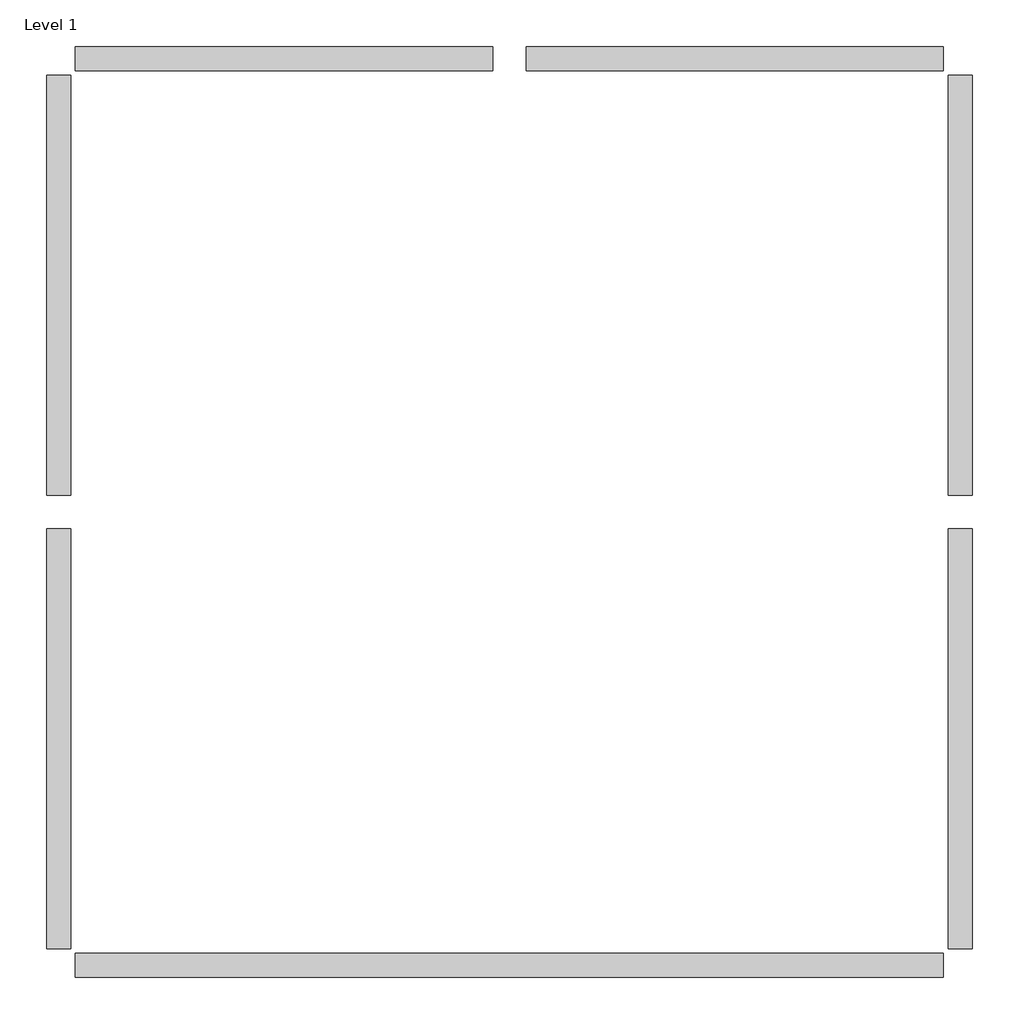
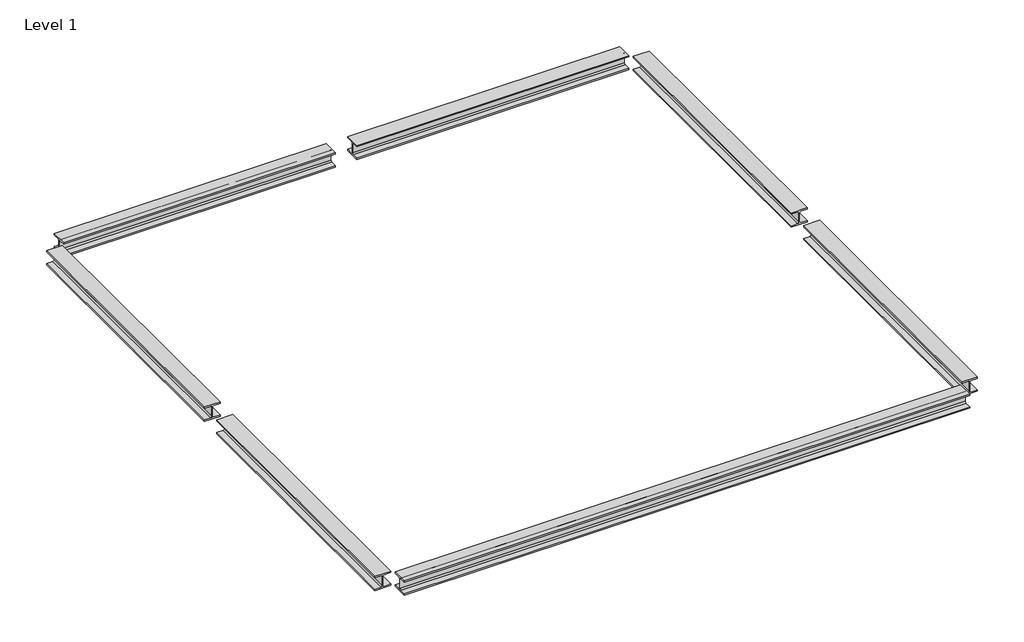
# One storey: 7 beams.
"""IFC4 building model written with IfcOpenShell, lengths in millimetres."""

import ifcopenshell
import ifcopenshell.guid

model = None  # the IFC model being written
_history = None  # IfcOwnerHistory: only IFC2X3 demands one
_inside = {}  # id of a spatial element -> (the spatial element, [elements in it])
_under = {}  # id of a project, library or spatial element -> (it, [spatial elements below it])
_declared = {}  # id of a project -> (the project, [libraries it declares])
_typed = {}  # id of a type object -> (the type object, [elements of that type])
_made_of = {}  # id of a material, layer set ... -> (it, [elements and type objects made of it])


def new_model(schema):
    """Start an empty IFC model of exactly this schema.

    Asked for "IFC4X3", IfcOpenShell would pick the latest addendum, in which some entities
    have other attributes; the version numbers below select the first issue.
    IFC2X3 requires an IfcOwnerHistory on every rooted entity: one is made here for all.
    """
    global model, _history
    if schema == "IFC4X3":
        model = ifcopenshell.file(schema_version=(4, 3, 0, 0))
    else:
        model = ifcopenshell.file(schema=schema)
    _inside.clear()
    _under.clear()
    _declared.clear()
    _typed.clear()
    _made_of.clear()
    _history = None
    if model.schema == "IFC2X3":
        org = make("IfcOrganization", Name="unknown")
        user = make(
            "IfcPersonAndOrganization",
            ThePerson=make("IfcPerson", FamilyName="unknown"),
            TheOrganization=org,
        )
        app = make(
            "IfcApplication",
            ApplicationDeveloper=org,
            Version="unknown",
            ApplicationFullName="unknown",
            ApplicationIdentifier="unknown",
        )
        _history = make(
            "IfcOwnerHistory",
            OwningUser=user,
            OwningApplication=app,
            ChangeAction="ADDED",
            CreationDate=0,
        )
    return model


def make(cls, **values):
    """One entity of the class cls with the attributes given. An attribute that is None is left unset."""
    return model.create_entity(
        cls, **{name: value for name, value in values.items() if value is not None}
    )


def rooted(cls, **values):
    """An entity with a GlobalId (a new one), such as an element, a storey or a relation."""
    return make(cls, GlobalId=ifcopenshell.guid.new(), OwnerHistory=_history, **values)


def si_unit(unit_type, name, prefix=None):
    """IfcSIUnit, for example si_unit("LENGTHUNIT", "METRE", prefix="MILLI")."""
    return make("IfcSIUnit", UnitType=unit_type, Prefix=prefix, Name=name)


def assignment(units):
    """IfcUnitAssignment: the units of a project."""
    return None if units is None else make("IfcUnitAssignment", Units=units)


def point(xyz):
    """IfcCartesianPoint."""
    return None if xyz is None else make("IfcCartesianPoint", Coordinates=xyz)


def direction(xyz):
    """IfcDirection."""
    return None if xyz is None else make("IfcDirection", DirectionRatios=xyz)


def frame(location, z_axis=None, x_axis=None):
    """IfcAxis2Placement3D, a coordinate frame: its origin and axes. An axis left out is left unset."""
    return make(
        "IfcAxis2Placement3D",
        Location=point(location),
        Axis=direction(z_axis),
        RefDirection=direction(x_axis),
    )


def frame_2d(location, x_axis=None):
    """IfcAxis2Placement2D, a coordinate frame in the plane: its origin and x axis."""
    return make(
        "IfcAxis2Placement2D", Location=point(location), RefDirection=direction(x_axis)
    )


def origin():
    """The frame at (0, 0, 0) with its axes left unset."""
    return frame((0.0, 0.0, 0.0))


def place(relative_to, where):
    """IfcLocalPlacement: puts the frame where relative to a parent placement (None: the world)."""
    return make(
        "IfcLocalPlacement", PlacementRelTo=relative_to, RelativePlacement=where
    )


def context(
    kind, dimensions, precision=None, world=None, true_north=None, identifier=None
):
    """IfcGeometricRepresentationContext, for example the 3D "Model" context."""
    return make(
        "IfcGeometricRepresentationContext",
        ContextIdentifier=identifier,
        ContextType=kind,
        CoordinateSpaceDimension=dimensions,
        Precision=precision,
        WorldCoordinateSystem=world,
        TrueNorth=true_north,
    )


def project(units=None, contexts=None):
    """IfcProject with its units and contexts."""
    return rooted(
        "IfcProject",
        Name="project",
        RepresentationContexts=contexts,
        UnitsInContext=assignment(units),
    )


def spatial(cls, under=None, at=None, **own):
    """A site, building, storey or space (cls), placed at a placement, below another one or the project."""
    s = rooted(cls, ObjectPlacement=at, **own)
    if under is not None:
        _under.setdefault(under.id(), (under, []))[1].append(s)
    return s


def polyline(points):
    """IfcPolyline through the points."""
    return make("IfcPolyline", Points=[point(p) for p in points])


def circle_curve(where, radius):
    """IfcCircle in the frame where."""
    return make("IfcCircle", Position=where, Radius=radius)


def trimmed(basis, trim1, trim2, sense, master):
    """IfcTrimmedCurve: the piece of a basis curve between two trims."""
    return make(
        "IfcTrimmedCurve",
        BasisCurve=basis,
        Trim1=trim1,
        Trim2=trim2,
        SenseAgreement=sense,
        MasterRepresentation=master,
    )


def segment(curve, same_sense, transition):
    """IfcCompositeCurveSegment."""
    return make(
        "IfcCompositeCurveSegment",
        Transition=transition,
        SameSense=same_sense,
        ParentCurve=curve,
    )


def composite_curve(segments, self_intersect=None):
    """IfcCompositeCurve: segments joined end to end."""
    return make("IfcCompositeCurve", Segments=segments, SelfIntersect=self_intersect)


def outline(outer, holes=None, kind="AREA"):
    """IfcArbitraryClosedProfileDef: a profile drawn as a closed curve; with holes, ...WithVoids."""
    if holes is None:
        return make("IfcArbitraryClosedProfileDef", ProfileType=kind, OuterCurve=outer)
    return make(
        "IfcArbitraryProfileDefWithVoids",
        ProfileType=kind,
        OuterCurve=outer,
        InnerCurves=holes,
    )


def extrude(swept, where, along, depth):
    """IfcExtrudedAreaSolid: the profile swept, set in the frame where, extruded along a direction by depth."""
    return make(
        "IfcExtrudedAreaSolid",
        SweptArea=swept,
        Position=where,
        ExtrudedDirection=direction(along),
        Depth=depth,
    )


def shape(context_of_items, identifier, shape_type, items):
    """IfcShapeRepresentation: the items that make up one representation, for example the "Body"."""
    return make(
        "IfcShapeRepresentation",
        ContextOfItems=context_of_items,
        RepresentationIdentifier=identifier,
        RepresentationType=shape_type,
        Items=items,
    )


def source(mapping_origin, context_of_items, identifier, shape_type, items):
    """IfcRepresentationMap: a shape defined once, which mapped items show again and again."""
    return make(
        "IfcRepresentationMap",
        MappingOrigin=mapping_origin,
        MappedRepresentation=shape(context_of_items, identifier, shape_type, items),
    )


def transform(
    local_origin,
    x_axis=None,
    y_axis=None,
    z_axis=None,
    scale=None,
    scale2=None,
    scale3=None,
    uniform=True,
):
    """IfcCartesianTransformationOperator3D, or its non-uniform kind. x_axis, y_axis, z_axis: its Axis1, 2, 3."""
    if uniform:
        return make(
            "IfcCartesianTransformationOperator3D",
            Axis1=direction(x_axis),
            Axis2=direction(y_axis),
            LocalOrigin=point(local_origin),
            Scale=scale,
            Axis3=direction(z_axis),
        )
    return make(
        "IfcCartesianTransformationOperator3DnonUniform",
        Axis1=direction(x_axis),
        Axis2=direction(y_axis),
        LocalOrigin=point(local_origin),
        Scale=scale,
        Axis3=direction(z_axis),
        Scale2=scale2,
        Scale3=scale3,
    )


def mapped(mapping_source, mapping_target):
    """IfcMappedItem: shows the shape of a source again, moved by a transform."""
    return make(
        "IfcMappedItem", MappingSource=mapping_source, MappingTarget=mapping_target
    )


def made_of(thing, what):
    """Note that an element or type object is made of a material, layer set ...; save() writes the relation."""
    if what is not None:
        _made_of.setdefault(what.id(), (what, []))[1].append(thing)
    return thing


def element(
    cls,
    number,
    at=None,
    inside=None,
    cuts=None,
    type_object=None,
    material=None,
    context=None,
    identifier="Body",
    shape_type=None,
    held_by="IfcProductDefinitionShape",
    body=None,
    shapes=None,
    **own,
):
    """One element of the class cls, such as IfcWall. Its Tag is "e" and its number.

    at: its placement. inside: the storey or other place that contains it. cuts: it is an
    opening in that element (IfcRelVoidsElement). A single representation is given by context,
    identifier, shape_type and body (its items); several are given by shapes. held_by: the class
    of the entity that holds the representations. save() writes the other relations.
    """
    e = rooted(cls, Tag="e%d" % number, ObjectPlacement=at, **own)
    if body is not None:
        shapes = [shape(context, identifier, shape_type, body)]
    if shapes is not None:
        e.Representation = make(held_by, Representations=shapes)
    if inside is not None:
        _inside.setdefault(inside.id(), (inside, []))[1].append(e)
    if cuts is not None:
        rooted(
            "IfcRelVoidsElement", RelatingBuildingElement=cuts, RelatedOpeningElement=e
        )
    if type_object is not None:
        _typed.setdefault(type_object.id(), (type_object, []))[1].append(e)
    return made_of(e, material)


def aggregate(whole, parts):
    """IfcRelAggregates: a whole, such as a stair, and the parts it consists of."""
    return rooted("IfcRelAggregates", RelatingObject=whole, RelatedObjects=parts)


def save(model, path):
    """Write the relations noted so far, then the file.

    IfcRelAggregates (storeys below a building ...), IfcRelContainedInSpatialStructure (elements
    in a storey), IfcRelDefinesByType, IfcRelAssociatesMaterial and IfcRelDeclares: one each for
    every whole, place, type object, material and project.
    """
    for whole, parts in _under.values():
        aggregate(whole, parts)
    for where, things in _inside.values():
        rooted(
            "IfcRelContainedInSpatialStructure",
            RelatedElements=things,
            RelatingStructure=where,
        )
    for kind, things in _typed.values():
        rooted("IfcRelDefinesByType", RelatedObjects=things, RelatingType=kind)
    for what, things in _made_of.values():
        rooted("IfcRelAssociatesMaterial", RelatedObjects=things, RelatingMaterial=what)
    for by, libraries in _declared.values():
        rooted("IfcRelDeclares", RelatingContext=by, RelatedDefinitions=libraries)
    model.write(path)


def parametric_beam_parametric_beam_2c295e66(model_context):
    return source(origin(), model_context, "Body", "SweptSolid", [
        extrude(outline(composite_curve([segment(polyline([(3.75, 72.0), (3.75, -72.0)]), True, "CONTINUOUS"), segment(trimmed(circle_curve(frame_2d((24.75, -72.0)), 21.0), [point((3.75, -72.0))], [point((24.75, -93.0))], True, "CARTESIAN"), True, "CONTINUOUS"), segment(polyline([(24.75, -93.0), (120.0, -93.0), (120.0, -115.0), (-120.0, -115.0), (-120.0, -93.0), (-24.75, -93.0)]), True, "CONTINUOUS"), segment(trimmed(circle_curve(frame_2d((-24.75, -72.0)), 21.0), [point((-24.75, -93.0))], [point((-3.75, -72.0))], True, "CARTESIAN"), True, "CONTINUOUS"), segment(polyline([(-3.75, -72.0), (-3.75, 72.0)]), True, "CONTINUOUS"), segment(trimmed(circle_curve(frame_2d((-24.75, 72.0)), 21.0), [point((-3.75, 72.0))], [point((-24.75, 93.0))], True, "CARTESIAN"), True, "CONTINUOUS"), segment(polyline([(-24.75, 93.0), (-120.0, 93.0), (-120.0, 115.0), (120.0, 115.0), (120.0, 93.0), (24.75, 93.0)]), True, "CONTINUOUS"), segment(trimmed(circle_curve(frame_2d((24.75, 72.0)), 21.0), [point((24.75, 93.0))], [point((3.75, 72.0))], True, "CARTESIAN"), True, "CONTINUOUS")], self_intersect=False)), frame((-4305.243318, 0.0, 0.0), z_axis=(1.0, 0.0, 0.0), x_axis=(0.0, 1.0, 0.0)), (0.0, 0.0, 1.0), 8610.486636),
    ])


def parametric_beam_parametric_beam_d4aa52de(model_context):
    return source(origin(), model_context, "Body", "SweptSolid", [
        extrude(outline(composite_curve([segment(polyline([(3.75, 72.0), (3.75, -72.0)]), True, "CONTINUOUS"), segment(trimmed(circle_curve(frame_2d((24.75, -72.0)), 21.0), [point((3.75, -72.0))], [point((24.75, -93.0))], True, "CARTESIAN"), True, "CONTINUOUS"), segment(polyline([(24.75, -93.0), (120.0, -93.0), (120.0, -115.0), (-120.0, -115.0), (-120.0, -93.0), (-24.75, -93.0)]), True, "CONTINUOUS"), segment(trimmed(circle_curve(frame_2d((-24.75, -72.0)), 21.0), [point((-24.75, -93.0))], [point((-3.75, -72.0))], True, "CARTESIAN"), True, "CONTINUOUS"), segment(polyline([(-3.75, -72.0), (-3.75, 72.0)]), True, "CONTINUOUS"), segment(trimmed(circle_curve(frame_2d((-24.75, 72.0)), 21.0), [point((-3.75, 72.0))], [point((-24.75, 93.0))], True, "CARTESIAN"), True, "CONTINUOUS"), segment(polyline([(-24.75, 93.0), (-120.0, 93.0), (-120.0, 115.0), (120.0, 115.0), (120.0, 93.0), (24.75, 93.0)]), True, "CONTINUOUS"), segment(trimmed(circle_curve(frame_2d((24.75, 72.0)), 21.0), [point((24.75, 93.0))], [point((3.75, 72.0))], True, "CARTESIAN"), True, "CONTINUOUS")], self_intersect=False)), frame((-2069.946659, 0.0, 0.0), z_axis=(1.0, 0.0, 0.0), x_axis=(0.0, 1.0, 0.0)), (0.0, 0.0, 1.0), 4139.893318),
    ])


def parametric_beam_parametric_beam_408cb472(model_context):
    return source(origin(), model_context, "Body", "SweptSolid", [
        extrude(outline(composite_curve([segment(polyline([(3.75, 72.0), (3.75, -72.0)]), True, "CONTINUOUS"), segment(trimmed(circle_curve(frame_2d((24.75, -72.0)), 21.0), [point((3.75, -72.0))], [point((24.75, -93.0))], True, "CARTESIAN"), True, "CONTINUOUS"), segment(polyline([(24.75, -93.0), (120.0, -93.0), (120.0, -115.0), (-120.0, -115.0), (-120.0, -93.0), (-24.75, -93.0)]), True, "CONTINUOUS"), segment(trimmed(circle_curve(frame_2d((-24.75, -72.0)), 21.0), [point((-24.75, -93.0))], [point((-3.75, -72.0))], True, "CARTESIAN"), True, "CONTINUOUS"), segment(polyline([(-3.75, -72.0), (-3.75, 72.0)]), True, "CONTINUOUS"), segment(trimmed(circle_curve(frame_2d((-24.75, 72.0)), 21.0), [point((-3.75, 72.0))], [point((-24.75, 93.0))], True, "CARTESIAN"), True, "CONTINUOUS"), segment(polyline([(-24.75, 93.0), (-120.0, 93.0), (-120.0, 115.0), (120.0, 115.0), (120.0, 93.0), (24.75, 93.0)]), True, "CONTINUOUS"), segment(trimmed(circle_curve(frame_2d((24.75, 72.0)), 21.0), [point((24.75, 93.0))], [point((3.75, 72.0))], True, "CARTESIAN"), True, "CONTINUOUS")], self_intersect=False)), frame((-2004.5455196, 0.0, 0.0), z_axis=(1.0, 0.0, 0.0), x_axis=(0.0, 1.0, 0.0)), (0.0, 0.0, 1.0), 4163.2589608),
    ])


model = new_model("IFC4")

# Units and contexts
model_context = context("Model", 3, world=origin())
ifc_project = project(units=[si_unit("LENGTHUNIT", "METRE", prefix="MILLI")], contexts=[model_context])

# Site, building, storey
site = spatial("IfcSite", under=ifc_project)
building = spatial("IfcBuilding", under=site)
storey = spatial("IfcBuildingStorey", under=building, Name="Level 1", Elevation=4000.0)

# Beams
placement = place(None, origin())
parametric_beam_parametric_beam_shape = parametric_beam_parametric_beam_2c295e66(model_context)
element("IfcBeam", 1, ObjectType="Parametric Beam : Parametric Beam", at=placement, inside=storey, context=model_context, shape_type="MappedRepresentation", body=[
    mapped(parametric_beam_parametric_beam_shape, transform((-492.9204879, -4027.830418, 3415.0), x_axis=(1.0, 0.0, 0.0), y_axis=(0.0, 1.0, 0.0), z_axis=(0.0, 0.0, 1.0))),
])
parametric_beam_parametric_beam_2_shape = parametric_beam_parametric_beam_d4aa52de(model_context)
element("IfcBeam", 2, ObjectType="Parametric Beam : Parametric Beam", at=placement, inside=storey, context=model_context, shape_type="MappedRepresentation", body=[
    mapped(parametric_beam_parametric_beam_2_shape, transform((1742.3761711, 4965.2875035, 3415.0), x_axis=(1.0, 0.0, 0.0), y_axis=(0.0, 1.0, 0.0), z_axis=(0.0, 0.0, 1.0))),
])
element("IfcBeam", 3, ObjectType="Parametric Beam : Parametric Beam", at=placement, inside=storey, context=model_context, shape_type="MappedRepresentation", body=[
    mapped(parametric_beam_parametric_beam_2_shape, transform((-2728.2171469, 4965.2875035, 3415.0), x_axis=(1.0, 0.0, 0.0), y_axis=(0.0, 1.0, 0.0), z_axis=(0.0, 0.0, 1.0))),
])
parametric_beam_parametric_beam_3_shape = parametric_beam_parametric_beam_408cb472(model_context)
element("IfcBeam", 4, ObjectType="Parametric Beam : Parametric Beam", at=placement, inside=storey, context=model_context, shape_type="MappedRepresentation", body=[
    mapped(parametric_beam_parametric_beam_3_shape, transform((-4963.5138059, -1702.4669769, 3415.0), x_axis=(0.0, -1.0, 0.0), y_axis=(1.0, 0.0, 0.0), z_axis=(0.0, 0.0, 1.0))),
])
element("IfcBeam", 5, ObjectType="Parametric Beam : Parametric Beam", at=placement, inside=storey, context=model_context, shape_type="MappedRepresentation", body=[
    mapped(parametric_beam_parametric_beam_3_shape, transform((-4963.5138059, 2794.0919839, 3415.0), x_axis=(0.0, -1.0, 0.0), y_axis=(1.0, 0.0, 0.0), z_axis=(0.0, 0.0, 1.0))),
])
element("IfcBeam", 6, ObjectType="Parametric Beam : Parametric Beam", at=placement, inside=storey, context=model_context, shape_type="MappedRepresentation", body=[
    mapped(parametric_beam_parametric_beam_3_shape, transform((3977.6728301, -1702.4669769, 3415.0), x_axis=(0.0, -1.0, 0.0), y_axis=(1.0, 0.0, 0.0), z_axis=(0.0, 0.0, 1.0))),
])
element("IfcBeam", 7, ObjectType="Parametric Beam : Parametric Beam", at=placement, inside=storey, context=model_context, shape_type="MappedRepresentation", body=[
    mapped(parametric_beam_parametric_beam_3_shape, transform((3977.6728301, 2794.0919839, 3415.0), x_axis=(0.0, -1.0, 0.0), y_axis=(1.0, 0.0, 0.0), z_axis=(0.0, 0.0, 1.0))),
])

save(model, "model.ifc")

# Revit data of these elements
# Type "Parametric Beam : Parametric Beam"
#   MHP_PRO_Name [instance default] = "HEA"
#   r [instance default] = 0.021 m
#   h [instance default] = 0.3 m
#   b [instance default] = 0.24 m
#   Tw [instance default] = 0.0075 m
#   Tf [instance default] = 0.012 m
#   Length [instance default] = 3 m
#   Viktor_Change [instance default] = yes
# Elements 1, 2, 3, 4, 5, 6, 7 (IfcBeam, "Parametric Beam : Parametric Beam")
#   MHP_PRO_Name = "HEA240"
#   r = 0.021 m
#   h = 0.23 m
#   b = 0.24 m
#   Tw = 0.0075 m
#   Tf = 0.022 m
#   Viktor_Change = no
#   Phase Created = New Construction
